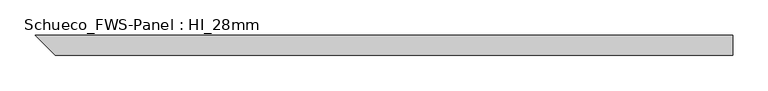
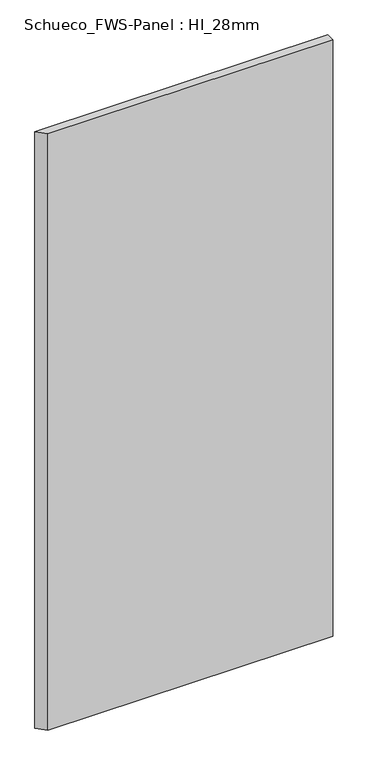
"""IFC4 building model written with IfcOpenShell, lengths in millimetres: plate geometry, Schueco_FWS-Panel : HI_28mm."""

from ifc_helpers import new_model, si_unit, origin, origin_with_axes, place, context, project, spatial, polyline, outline, extrude, source, transform, mapped, element, save


def schueco_fws_panel_hi_28mm_c7e54ee3(model_context):
    return source(origin(), model_context, "Body", "SweptSolid", [
        extrude(outline(polyline([(-494.5, 0.0), (494.5, 0.0), (494.5, -28.0), (-466.5, -28.0), (-494.5, 0.0)])), origin_with_axes(), (0.0, 0.0, 1.0), 2128.0),
    ])


if __name__ == "__main__":
    model = new_model("IFC4")
    model_context = context("Model", 3, world=origin())
    ifc_project = project(units=[si_unit("LENGTHUNIT", "METRE", prefix="MILLI")], contexts=[model_context])
    site = spatial("IfcSite", under=ifc_project)
    building = spatial("IfcBuilding", under=site)
    placement = place(None, origin())
    schueco_fws_panel_hi_28mm_shape = schueco_fws_panel_hi_28mm_c7e54ee3(model_context)
    element("IfcPlate", 1, ObjectType="Schueco_FWS-Panel : HI_28mm", at=placement, inside=building, context=model_context, shape_type="MappedRepresentation", body=[
        mapped(schueco_fws_panel_hi_28mm_shape, transform((0.0, 0.0, 0.0), x_axis=(1.0, 0.0, 0.0), y_axis=(0.0, 1.0, 0.0), z_axis=(0.0, 0.0, 1.0))),
    ])
    save(model, "model.ifc")

# Revit data of these elements
# Type "Schueco_FWS-Panel : HI_28mm"
#   Model = "Panel 28mm"
#   Manufacturer = "Schueco International KG"
#   Analytic Construction = "<Keine Auswahl>"
#   Panel thickness = 28 mm
#   Angle right [instance default] = 0.00°
#   Angle left [instance default] = 0.00°
#   AR [instance default] = 0.00°
#   AL [instance default] = 0.00°
#   FWS SI insert unit = no
#   FWS HI insert unit = yes
#   Det_R [instance default] = yes
#   Det_L [instance default] = yes
#   Panel = Alu
# Element 1 (IfcPlate, "Schueco_FWS-Panel : HI_28mm")
#   Angle left = 45.00°
#   AL = 45.00°
#   Det_L = no
#   Materials on its faces: "Alu"
# Materials
#   "Alu": class "Glas", colour RGB 140 140 140, transparency 0
